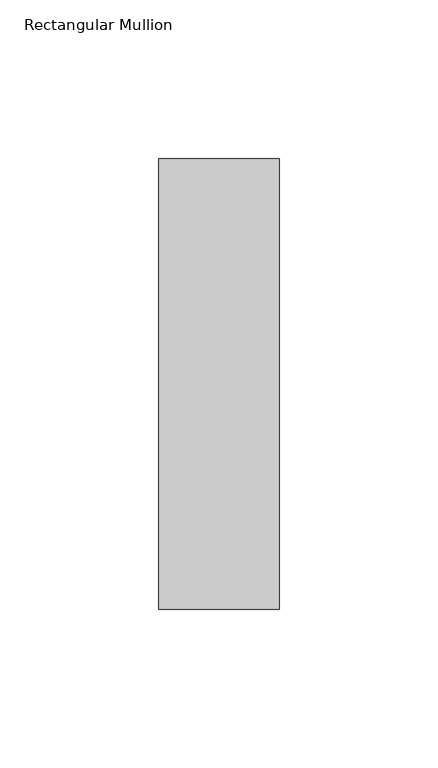
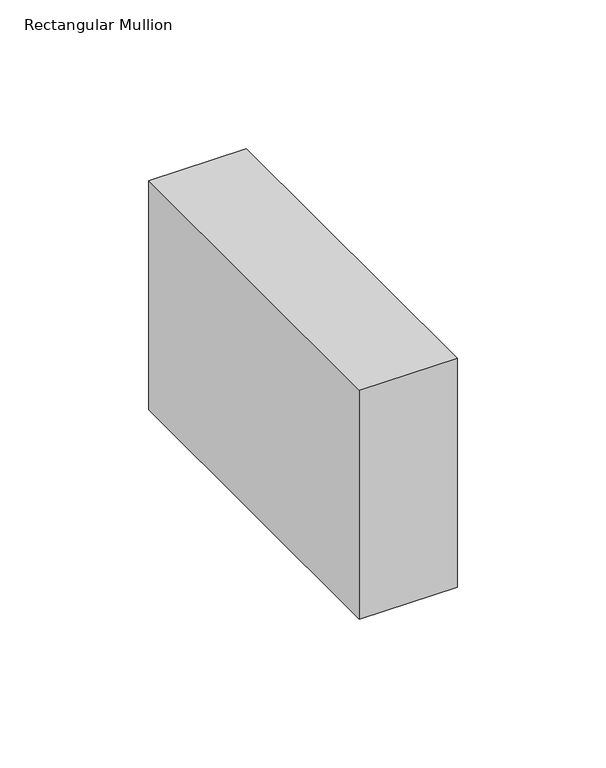
"""IFC4 building model written with IfcOpenShell, lengths in millimetres: member geometry, Rectangular Mullion : NLRS_21_CWM_hsb-regel 38x142_gen_rsf."""

from ifc_helpers import new_model, si_unit, frame, origin, place, context, project, spatial, polyline, outline, extrude, source, transform, mapped, element, save


def rectangular_mullion_ff2f71bd(model_context):
    return source(origin(), model_context, "Body", "SweptSolid", [
        extrude(outline(polyline([(0.0, -71.0), (-38.0, -71.0), (-38.0, 71.0), (0.0, 71.0), (0.0, -71.0)])), frame((0.0, 0.0, -94.1558939), z_axis=(0.0, 0.0, 1.0), x_axis=(1.0, 0.0, 0.0)), (0.0, 0.0, 1.0), 94.1558939),
    ])


if __name__ == "__main__":
    model = new_model("IFC4")
    model_context = context("Model", 3, world=origin())
    ifc_project = project(units=[si_unit("LENGTHUNIT", "METRE", prefix="MILLI")], contexts=[model_context])
    site = spatial("IfcSite", under=ifc_project)
    building = spatial("IfcBuilding", under=site)
    placement = place(None, origin())
    rectangular_mullion_shape = rectangular_mullion_ff2f71bd(model_context)
    element("IfcMember", 1, ObjectType="Rectangular Mullion : NLRS_21_CWM_hsb-regel 38x142_gen_rsf", at=placement, inside=building, context=model_context, shape_type="MappedRepresentation", body=[
        mapped(rectangular_mullion_shape, transform((0.0, 0.0, 0.0), x_axis=(1.0, 0.0, 0.0), y_axis=(0.0, 1.0, 0.0), z_axis=(0.0, 0.0, 1.0))),
    ])
    save(model, "model.ifc")

# Revit data of these elements
# Type "Rectangular Mullion : NLRS_21_CWM_hsb-regel 38x142_gen_rsf"
#   Export Type to IFC As = "IfcWall"
#   Type IfcGUID = "07M7mRoiH1CR8m_RSKIwpF"
#   Assembly Code = "21.10"
#   built-in parameter 1007322 = 0.465879 (stored number, unit not read)
#   built-in parameter 1007321 = 0.062336 (stored number, unit not read)
#   built-in parameter 1007320 = 0.062336 (stored number, unit not read)
# Element 1 (IfcMember, "Rectangular Mullion : NLRS_21_CWM_hsb-regel 38x142_gen_rsf")
#   Materials on its faces: "NLRS_i2_hout naaldhout vuren_gen_rsf"
# Materials
#   "NLRS_i2_hout naaldhout vuren_gen_rsf": class "I - Hout", colour RGB 234 199 147, transparency 0, Keynote = "i2", Manufacturer = "Revit Standards Foundation", URL = "www.revitstandards.org", Description = "hout vuren", Cost = 0
